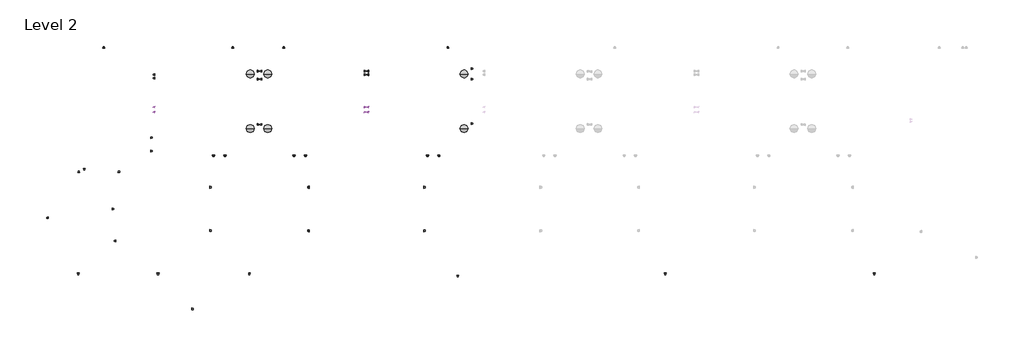
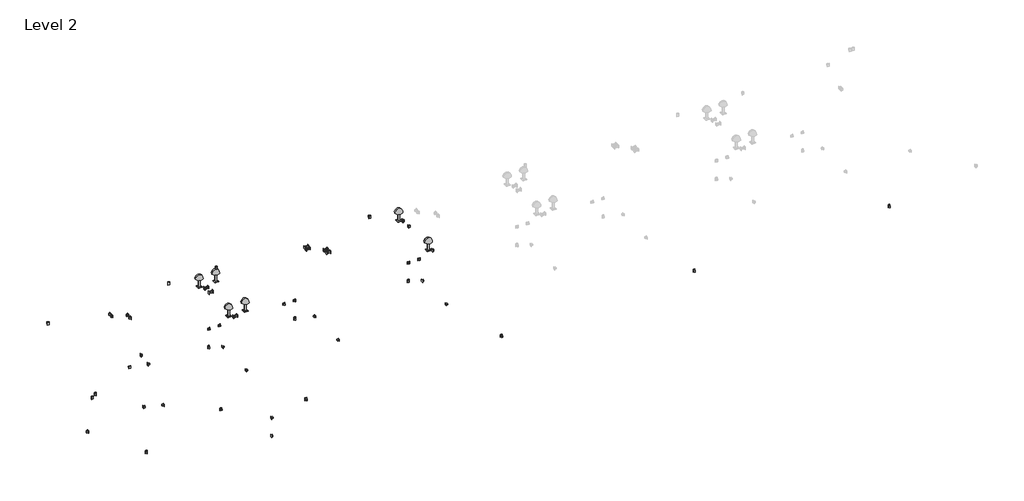
# One storey, part 1 of 2: 40 proxies, 16 switching devices, 6 light fixtures.
# Revit data of these elements (continued)
# Type "Table Lamp - Hemispheric : 60W - 230V" (continued)
#   built-in parameter 1150137 = 1
#   Color Filter = 16777215
#   Ballast Number of Poles = 1
#   T.L. Material = Wood - Birch
#   Mount Material = Metal - Chrome
#   Load Classification = Lighting - Dwelling Unit
#   Shade Material = Glass - Frosted
#   Base Material = Wood - Birch
#   Dimming Lamp Color Temperature Shift = (empty or 0)
#   Default Elevation = 0
#   Wattage Comments = ""
# Type "Lighting Switches One Way : One Way Switch"
#   Type Mark = "Lighting Switches One Way"
#   Classification.OmniClass.21.Number = "21-04 50 40 10"
#   Classification.OmniClass.21.Description = "Lighting Control"
#   Classification.UniFormat.II.Description = "Lighting Control"
#   Classification.OmniClass.23.Number = "23-35 37 00"
#   Classification.OmniClass.23.Description = "Electrical Switches"
#   Classification.UniFormat.II.Number = "D5040.10"
#   COBie.Type.CreatedBy = "info@mma.ie"
#   COBie.Type.CreatedOn = "2017-07-25T10:15:16"
#   COBie.Type.Name = "Lighting Switches One Way"
#   COBie.Type.Category = "23-35 37 00 : Electrical Switches"
#   COBie.Type.Description = "Lighting Switches One Way_One Way Switch"
#   COBie.Type.AssetType = "Fixed"
#   COBie.Type.Manufacturer = ""
#   COBie.Type.ModelNumber = ""
#   Label = ""
#   Keynote = "26 36 13.A"
#   COBie.Type.ReplacementCost = 0
#   Switch Voltage [instance default] = 230 V
#   Default Elevation = 1200 mm
#   Apparent Load = 0 VA
#   1.W.S. Width = 86 mm
#   1.W.S. Height = 86 mm
#   1.W.S. Depth = 59 mm
#   COBie.Type = yes
#   Visibility 7 = no
#   Visibility 6 = no
#   Visibility 5 = yes
#   Visibility 4 = no
#   Visibility 3 = no
#   Visibility 2 = no
#   Visibility 1 = no
#   Ballast Number of Poles = 1
#   Load Classification = Other
#   1.W.S. Material = Metal - Chrome
# Type "Lighting Switches Two Way : Two Way Switch"
#   Type Mark = "Lighting Switches Two Way"
#   Classification.OmniClass.23.Number = "23-35 37 00"
#   Classification.OmniClass.23.Description = "Electrical Switches"
#   COBie.Type.CreatedBy = "info@mma.ie"
#   COBie.Type.CreatedOn = "2017-07-25T10:15:16"
#   COBie.Type.Name = "Lighting Switches Two Way"
#   COBie.Type.Category = "23-35 37 00 : Electrical Switches"
#   COBie.Type.Description = "Lighting Switches Two Way_Two Way Switch"
#   COBie.Type.AssetType = "Fixed"
#   COBie.Type.Manufacturer = ""
#   COBie.Type.ModelNumber = ""
#   Label = ""
#   Keynote = "26 36 13.B"
#   COBie.Type.ReplacementCost = 0
#   Switch Voltage [instance default] = 230 V
#   Default Elevation = 1200 mm
#   Apparent Load = 0 VA
#   2.W.S. Width = 86 mm
#   2.W.S. Height = 86 mm
#   2.W.S. Depth = 59 mm
#   COBie.Type = yes
#   Visibility 7 = no
#   Visibility 6 = no
#   Visibility 5 = yes
#   Visibility 4 = no
#   Visibility 3 = no
#   Visibility 2 = no
#   Visibility 1 = no
#   Ballast Number of Poles = 1
#   Load Classification = Other
#   2.W.S. Material = Metal - Chrome
# Element 1 (IfcBuildingElementProxy, "M_Duplex Receptacle - Top Switched : Standard")
#   Mark = "7"
#   COBie.CreatedBy = "info@mma.ie"
#   COBie.CreatedOn = "2017-07-25T10:15:16"
#   COBie.Component.Name = "M_Duplex Receptacle - Top Switched_7"
#   COBie.Component.Space = "207"
#   COBie.Component.Description = "M_Duplex Receptacle - Top Switched: Standard"
#   Notes = "n/a"
#   COBie = yes
#   Phase Created = New Construction
# Element 2 (IfcBuildingElementProxy, "M_Duplex Receptacle - Top Switched : Standard")
#   Mark = "8"
#   COBie.CreatedBy = "info@mma.ie"
#   COBie.CreatedOn = "2017-07-25T10:15:16"
#   COBie.Component.Name = "M_Duplex Receptacle - Top Switched_8"
#   COBie.Component.Space = "207"
#   COBie.Component.Description = "M_Duplex Receptacle - Top Switched: Standard"
#   Notes = "n/a"
#   COBie = yes
#   Phase Created = New Construction
# Element 3 (IfcBuildingElementProxy, "M_Duplex Receptacle - Top Switched : Standard")
#   Mark = "9"
#   COBie.CreatedBy = "info@mma.ie"
#   COBie.CreatedOn = "2017-07-25T10:15:16"
#   COBie.Component.Name = "M_Duplex Receptacle - Top Switched_9"
#   COBie.Component.Space = "205"
#   COBie.Component.Description = "M_Duplex Receptacle - Top Switched: Standard"
#   Notes = "n/a"
#   COBie = yes
#   Phase Created = New Construction
# Element 4 (IfcBuildingElementProxy, "M_Duplex Receptacle - Top Switched : Standard")
#   Mark = "10"
#   COBie.CreatedBy = "info@mma.ie"
#   COBie.CreatedOn = "2017-07-25T10:15:16"
#   COBie.Component.Name = "M_Duplex Receptacle - Top Switched_10"
#   COBie.Component.Space = "205"
#   COBie.Component.Description = "M_Duplex Receptacle - Top Switched: Standard"
#   Notes = "n/a"
#   COBie = yes
#   Phase Created = New Construction
# Element 5 (IfcBuildingElementProxy, "M_Duplex Receptacle - Top Switched : Standard")
#   Mark = "15"
#   COBie.CreatedBy = "info@mma.ie"
#   COBie.CreatedOn = "2017-07-25T10:15:16"
#   COBie.Component.Name = "M_Duplex Receptacle - Top Switched_15"
#   COBie.Component.Space = "203"
#   COBie.Component.Description = "M_Duplex Receptacle - Top Switched: Standard"
#   Notes = "n/a"
#   COBie = yes
#   Phase Created = New Construction
# Element 6 (IfcBuildingElementProxy, "M_Duplex Receptacle - Top Switched : Standard")
#   Mark = "16"
#   COBie.CreatedBy = "info@mma.ie"
#   COBie.CreatedOn = "2017-07-25T10:15:16"
#   COBie.Component.Name = "M_Duplex Receptacle - Top Switched_16"
#   COBie.Component.Space = "203"
#   COBie.Component.Description = "M_Duplex Receptacle - Top Switched: Standard"
#   Notes = "n/a"
#   COBie = yes
#   Phase Created = New Construction
# Element 7 (IfcBuildingElementProxy, "M_Receptacle - 220V : Standard")
#   Mark = "15"
#   COBie.CreatedBy = "info@mma.ie"
#   COBie.CreatedOn = "2017-07-25T10:15:16"
#   COBie.Component.Name = "M_Receptacle - 220V_15"
#   COBie.Component.Space = "207"
#   COBie.Component.Description = "M_Receptacle - 220V: Standard"
#   Notes = "n/a"
#   COBie = yes
#   Phase Created = New Construction
# Element 8 (IfcBuildingElementProxy, "M_Receptacle - 220V : Standard")
#   Mark = "16"
#   COBie.CreatedBy = "info@mma.ie"
#   COBie.CreatedOn = "2017-07-25T10:15:16"
#   COBie.Component.Name = "M_Receptacle - 220V_16"
#   COBie.Component.Space = "207"
#   COBie.Component.Description = "M_Receptacle - 220V: Standard"
#   Notes = "n/a"
#   COBie = yes
#   Phase Created = New Construction
# Element 9 (IfcBuildingElementProxy, "M_Receptacle - 220V : Standard")
#   Mark = "17"
#   COBie.CreatedBy = "info@mma.ie"
#   COBie.CreatedOn = "2017-07-25T10:15:16"
#   COBie.Component.Name = "M_Receptacle - 220V_17"
#   COBie.Component.Space = "207"
#   COBie.Component.Description = "M_Receptacle - 220V: Standard"
#   Notes = "n/a"
#   COBie = yes
#   Phase Created = New Construction
# Element 10 (IfcBuildingElementProxy, "M_Receptacle - 220V : Standard")
#   Mark = "18"
#   COBie.CreatedBy = "info@mma.ie"
#   COBie.CreatedOn = "2017-07-25T10:15:16"
#   COBie.Component.Name = "M_Receptacle - 220V_18"
#   COBie.Component.Space = "207"
#   COBie.Component.Description = "M_Receptacle - 220V: Standard"
#   Notes = "n/a"
#   COBie = yes
#   Phase Created = New Construction
# Element 11 (IfcBuildingElementProxy, "M_Receptacle - 220V : Standard")
#   Mark = "19"
#   COBie.CreatedBy = "info@mma.ie"
#   COBie.CreatedOn = "2017-07-25T10:15:16"
#   COBie.Component.Name = "M_Receptacle - 220V_19"
#   COBie.Component.Space = "205"
#   COBie.Component.Description = "M_Receptacle - 220V: Standard"
#   Notes = "n/a"
#   COBie = yes
#   Phase Created = New Construction
# Element 12 (IfcBuildingElementProxy, "M_Receptacle - 220V : Standard")
#   Mark = "20"
#   COBie.CreatedBy = "info@mma.ie"
#   COBie.CreatedOn = "2017-07-25T10:15:16"
#   COBie.Component.Name = "M_Receptacle - 220V_20"
#   COBie.Component.Space = "203"
#   COBie.Component.Description = "M_Receptacle - 220V: Standard"
#   Notes = "n/a"
#   COBie = yes
#   Phase Created = New Construction
# Element 13 (IfcBuildingElementProxy, "M_Receptacle - 220V : Standard")
#   Mark = "21"
#   COBie.CreatedBy = "info@mma.ie"
#   COBie.CreatedOn = "2017-07-25T10:15:16"
#   COBie.Component.Name = "M_Receptacle - 220V_21"
#   COBie.Component.Space = "205"
#   COBie.Component.Description = "M_Receptacle - 220V: Standard"
#   Notes = "n/a"
#   COBie = yes
#   Phase Created = New Construction
# Element 14 (IfcBuildingElementProxy, "M_Receptacle - 220V : Standard")
#   Mark = "22"
#   COBie.CreatedBy = "info@mma.ie"
#   COBie.CreatedOn = "2017-07-25T10:15:16"
#   COBie.Component.Name = "M_Receptacle - 220V_22"
#   COBie.Component.Space = "203"
#   COBie.Component.Description = "M_Receptacle - 220V: Standard"
#   Notes = "n/a"
#   COBie = yes
#   Phase Created = New Construction
# Element 15 (IfcBuildingElementProxy, "M_Receptacle - 220V : Standard")
#   Comments = ""
#   Mark = "23"
#   COBie.CreatedBy = "info@mma.ie"
#   COBie.CreatedOn = "2017-07-25T10:15:16"
#   COBie.Component.Name = "M_Receptacle - 220V_23"
#   COBie.Component.Space = "202"
#   COBie.Component.Description = "M_Receptacle - 220V: Standard"
#   Notes = "n/a"
#   COBie = yes
#   Phase Created = New Construction
# Element 16 (IfcBuildingElementProxy, "M_Receptacle - 220V : Standard")
#   Mark = "24"
#   COBie.CreatedBy = "info@mma.ie"
#   COBie.CreatedOn = "2017-07-25T10:15:16"
#   COBie.Component.Name = "M_Receptacle - 220V_24"
#   COBie.Component.Space = "203"
#   COBie.Component.Description = "M_Receptacle - 220V: Standard"
#   Notes = "n/a"
#   COBie = yes
#   Phase Created = New Construction
# Element 17 (IfcBuildingElementProxy, "M_Receptacle - 220V : Standard")
#   Mark = "25"
#   COBie.CreatedBy = "info@mma.ie"
#   COBie.CreatedOn = "2017-07-25T10:15:16"
#   COBie.Component.Name = "M_Receptacle - 220V_25"
#   COBie.Component.Space = "203"
#   COBie.Component.Description = "M_Receptacle - 220V: Standard"
#   Notes = "n/a"
#   COBie = yes
#   Phase Created = New Construction
# Element 18 (IfcBuildingElementProxy, "M_Receptacle - 220V : Standard")
#   Comments = ""
#   Mark = "26"
#   COBie.CreatedBy = "info@mma.ie"
#   COBie.CreatedOn = "2017-07-25T10:15:16"
#   COBie.Component.Name = "M_Receptacle - 220V_26"
#   COBie.Component.Space = "202"
#   COBie.Component.Description = "M_Receptacle - 220V: Standard"
#   Notes = "n/a"
#   COBie = yes
#   Phase Created = New Construction
# Element 19 (IfcBuildingElementProxy, "M_Receptacle - 220V : Standard")
#   Comments = ""
#   Mark = "27"
#   COBie.CreatedBy = "info@mma.ie"
#   COBie.CreatedOn = "2017-07-25T10:15:16"
#   COBie.Component.Name = "M_Receptacle - 220V_27"
#   COBie.Component.Space = "202"
#   COBie.Component.Description = "M_Receptacle - 220V: Standard"
#   Notes = "n/a"
#   COBie = yes
#   Phase Created = New Construction
# Element 20 (IfcBuildingElementProxy, "M_Receptacle - 220V : Standard")
#   Mark = "28"
#   COBie.CreatedBy = "info@mma.ie"
#   COBie.CreatedOn = "2017-07-25T10:15:16"
#   COBie.Component.Name = "M_Receptacle - 220V_28"
#   COBie.Component.Space = "201"
#   COBie.Component.Description = "M_Receptacle - 220V: Standard"
#   Notes = "n/a"
#   COBie = yes
#   Phase Created = New Construction
# Element 21 (IfcBuildingElementProxy, "M_Receptacle - 220V : Standard")
#   Mark = "29"
#   COBie.CreatedBy = "info@mma.ie"
#   COBie.CreatedOn = "2017-07-25T10:15:16"
#   COBie.Component.Name = "M_Receptacle - 220V_29"
#   COBie.Component.Space = "201"
#   COBie.Component.Description = "M_Receptacle - 220V: Standard"
#   Notes = "n/a"
#   COBie = yes
#   Phase Created = New Construction
# Element 22 (IfcBuildingElementProxy, "M_Receptacle - 220V : Standard")
#   Mark = "30"
#   COBie.CreatedBy = "info@mma.ie"
#   COBie.CreatedOn = "2017-07-25T10:15:16"
#   COBie.Component.Name = "M_Receptacle - 220V_30"
#   COBie.Component.Space = "201"
#   COBie.Component.Description = "M_Receptacle - 220V: Standard"
#   Notes = "n/a"
#   COBie = yes
#   Phase Created = New Construction
# Element 23 (IfcBuildingElementProxy, "M_Receptacle - 220V : Standard")
#   Mark = "31"
#   COBie.CreatedBy = "info@mma.ie"
#   COBie.CreatedOn = "2017-07-25T10:15:16"
#   COBie.Component.Name = "M_Receptacle - 220V_31"
#   COBie.Component.Space = "201"
#   COBie.Component.Description = "M_Receptacle - 220V: Standard"
#   Notes = "n/a"
#   COBie = yes
#   Phase Created = New Construction
# Element 24 (IfcBuildingElementProxy, "M_Receptacle - 220V : Standard")
#   Mark = "32"
#   COBie.CreatedBy = "info@mma.ie"
#   COBie.CreatedOn = "2017-07-25T10:15:16"
#   COBie.Component.Name = "M_Receptacle - 220V_32"
#   COBie.Component.Space = "218"
#   COBie.Component.Description = "M_Receptacle - 220V: Standard"
#   Notes = "n/a"
#   COBie = yes
#   Phase Created = New Construction
# Element 25 (IfcBuildingElementProxy, "M_Receptacle - 220V : Standard")
#   Mark = "33"
#   COBie.CreatedBy = "info@mma.ie"
#   COBie.CreatedOn = "2017-07-25T10:15:16"
#   COBie.Component.Name = "M_Receptacle - 220V_33"
#   COBie.Component.Space = "217"
#   COBie.Component.Description = "M_Receptacle - 220V: Standard"
#   Notes = "n/a"
#   COBie = yes
#   Phase Created = New Construction
# Element 26 (IfcBuildingElementProxy, "M_Receptacle - 220V : Standard")
#   Mark = "34"
#   COBie.CreatedBy = "info@mma.ie"
#   COBie.CreatedOn = "2017-07-25T10:15:16"
#   COBie.Component.Name = "M_Receptacle - 220V_34"
#   COBie.Component.Space = "217"
#   COBie.Component.Description = "M_Receptacle - 220V: Standard"
#   Notes = "n/a"
#   COBie = yes
#   Phase Created = New Construction
# Element 27 (IfcBuildingElementProxy, "M_Receptacle - 220V : Standard")
#   Mark = "35"
#   COBie.CreatedBy = "info@mma.ie"
#   COBie.CreatedOn = "2017-07-25T10:15:16"
#   COBie.Component.Name = "M_Receptacle - 220V_35"
#   COBie.Component.Space = "217"
#   COBie.Component.Description = "M_Receptacle - 220V: Standard"
#   Notes = "n/a"
#   COBie = yes
#   Phase Created = New Construction
# Element 28 (IfcBuildingElementProxy, "M_Receptacle - 220V : Standard")
#   Mark = "36"
#   COBie.CreatedBy = "info@mma.ie"
#   COBie.CreatedOn = "2017-07-25T10:15:16"
#   COBie.Component.Name = "M_Receptacle - 220V_36"
#   COBie.Component.Space = "217"
#   COBie.Component.Description = "M_Receptacle - 220V: Standard"
#   Notes = "n/a"
#   COBie = yes
#   Phase Created = New Construction
# Element 29 (IfcBuildingElementProxy, "M_Receptacle - 220V : Standard")
#   Mark = "80"
#   COBie.CreatedBy = "info@mma.ie"
#   COBie.CreatedOn = "2017-07-25T10:15:16"
#   COBie.Component.Name = "M_Receptacle - 220V_80"
#   COBie.Component.Space = "205"
#   COBie.Component.Description = "M_Receptacle - 220V: Standard"
#   Notes = "n/a"
#   COBie = yes
#   Phase Created = New Construction
# Element 30 (IfcBuildingElementProxy, "M_Receptacle - 220V : Standard")
#   Mark = "81"
#   COBie.CreatedBy = "info@mma.ie"
#   COBie.CreatedOn = "2017-07-25T10:15:16"
#   COBie.Component.Name = "M_Receptacle - 220V_81"
#   COBie.Component.Space = "205"
#   COBie.Component.Description = "M_Receptacle - 220V: Standard"
#   Notes = "n/a"
#   COBie = yes
#   Phase Created = New Construction
# Element 31 (IfcBuildingElementProxy, "M_Receptacle - DATA socket : Standard")
#   Mark = "1"
#   COBie.CreatedBy = "info@mma.ie"
#   COBie.CreatedOn = "2017-07-25T10:15:16"
#   COBie.Component.Name = "M_Receptacle - DATA socket_1"
#   COBie.Component.Space = "203"
#   COBie.Component.Description = "M_Receptacle - DATA socket: Standard"
#   Notes = "n/a"
#   COBie = yes
#   Phase Created = New Construction
# Element 32 (IfcBuildingElementProxy, "M_Receptacle - DATA socket : Standard")
#   Comments = ""
#   Mark = "2"
#   COBie.CreatedBy = "info@mma.ie"
#   COBie.CreatedOn = "2017-07-25T10:15:16"
#   COBie.Component.Name = "M_Receptacle - DATA socket_2"
#   COBie.Component.Space = "202"
#   COBie.Component.Description = "M_Receptacle - DATA socket: Standard"
#   Notes = "n/a"
#   COBie = yes
#   Phase Created = New Construction
# Element 33 (IfcBuildingElementProxy, "M_Receptacle - DATA socket : Standard")
#   Mark = "3"
#   COBie.CreatedBy = "info@mma.ie"
#   COBie.CreatedOn = "2017-07-25T10:15:16"
#   COBie.Component.Name = "M_Receptacle - DATA socket_3"
#   COBie.Component.Space = "203"
#   COBie.Component.Description = "M_Receptacle - DATA socket: Standard"
#   Notes = "n/a"
#   COBie = yes
#   Phase Created = New Construction
# Element 34 (IfcBuildingElementProxy, "M_Receptacle - DATA socket : Standard")
#   Mark = "4"
#   COBie.CreatedBy = "info@mma.ie"
#   COBie.CreatedOn = "2017-07-25T10:15:16"
#   COBie.Component.Name = "M_Receptacle - DATA socket_4"
#   COBie.Component.Space = "205"
#   COBie.Component.Description = "M_Receptacle - DATA socket: Standard"
#   Notes = "n/a"
#   COBie = yes
#   Phase Created = New Construction
# Element 35 (IfcBuildingElementProxy, "M_Receptacle - DATA socket : Standard")
#   Mark = "5"
#   COBie.CreatedBy = "info@mma.ie"
#   COBie.CreatedOn = "2017-07-25T10:15:16"
#   COBie.Component.Name = "M_Receptacle - DATA socket_5"
#   COBie.Component.Space = "207"
#   COBie.Component.Description = "M_Receptacle - DATA socket: Standard"
#   Notes = "n/a"
#   COBie = yes
#   Phase Created = New Construction
# Element 36 (IfcBuildingElementProxy, "M_Receptacle - DATA socket : Standard")
#   Mark = "19"
#   COBie.CreatedBy = "info@mma.ie"
#   COBie.CreatedOn = "2017-07-25T10:15:16"
#   COBie.Component.Name = "M_Receptacle - DATA socket_19"
#   COBie.Component.Space = "205"
#   COBie.Component.Description = "M_Receptacle - DATA socket: Standard"
#   Notes = "n/a"
#   COBie = yes
#   Phase Created = New Construction
# Element 37 (IfcBuildingElementProxy, "M_Receptacle - DATA socket : Standard")
#   Mark = "20"
#   COBie.CreatedBy = "info@mma.ie"
#   COBie.CreatedOn = "2017-07-25T10:15:16"
#   COBie.Component.Name = "M_Receptacle - DATA socket_20"
#   COBie.Component.Space = "207"
#   COBie.Component.Description = "M_Receptacle - DATA socket: Standard"
#   Notes = "n/a"
#   COBie = yes
#   Phase Created = New Construction
# Element 38 (IfcBuildingElementProxy, "M_Receptacle -TV /Satellite Socket : Standard")
#   Mark = "1"
#   COBie.CreatedBy = "info@mma.ie"
#   COBie.CreatedOn = "2017-07-25T10:15:16"
#   COBie.Component.Name = "M_Receptacle -TV_1"
#   COBie.Component.Space = "207"
#   COBie.Component.Description = "M_Receptacle -TV: Standard"
#   Notes = "n/a"
#   COBie = yes
#   Phase Created = New Construction
# Element 39 (IfcBuildingElementProxy, "M_Receptacle -TV /Satellite Socket : Standard")
#   Mark = "2"
#   COBie.CreatedBy = "info@mma.ie"
#   COBie.CreatedOn = "2017-07-25T10:15:16"
#   COBie.Component.Name = "M_Receptacle -TV_2"
#   COBie.Component.Space = "203"
#   COBie.Component.Description = "M_Receptacle -TV: Standard"
#   Notes = "n/a"
#   COBie = yes
#   Phase Created = New Construction
# Element 40 (IfcBuildingElementProxy, "M_Receptacle -TV /Satellite Socket : Standard")
#   Mark = "7"
#   COBie.CreatedBy = "info@mma.ie"
#   COBie.CreatedOn = "2017-07-25T10:15:16"
#   COBie.Component.Name = "M_Receptacle -TV_7"
#   COBie.Component.Space = "205"
#   COBie.Component.Description = "M_Receptacle -TV: Standard"
#   Notes = "n/a"
#   COBie = yes
#   Phase Created = New Construction
# Element 41 (IfcLightFixture, "Table Lamp - Hemispheric : 60W - 230V")
#   Comments = "Lamps"
#   Mark = "5"
#   COBie.ExternalIdentifier = ""
#   COBie.CreatedBy = "info@mma.ie"
#   COBie.CreatedOn = "2017-07-25T10:15:16"
#   COBie.Component.Name = "Table Lamp - Hemispheric_5"
#   COBie.Component.Space = "207"
#   COBie.Component.Description = "Table Lamp - Hemispheric: 60W - 230V"
#   Notes = "n/a"
#   Floor Level = "Level 2"
#   COBie = yes
#   Phase Created = New Construction
#   Materials on its faces: "Metal - Chrome", "Glass - Frosted", "Wood - Birch"
# Element 42 (IfcLightFixture, "Table Lamp - Hemispheric : 60W - 230V")
#   Comments = "Lamps"
#   Mark = "6"
#   COBie.CreatedBy = "info@mma.ie"
#   COBie.CreatedOn = "2017-07-25T10:15:16"
#   COBie.Component.Name = "Table Lamp - Hemispheric_6"
#   COBie.Component.Space = "207"
#   COBie.Component.Description = "Table Lamp - Hemispheric: 60W - 230V"
#   Notes = "n/a"
#   Floor Level = "Level 2"
#   COBie = yes
#   Phase Created = New Construction
#   Materials on its faces: "Metal - Chrome", "Glass - Frosted", "Wood - Birch"
# Element 43 (IfcLightFixture, "Table Lamp - Hemispheric : 60W - 230V")
#   Comments = "Lamps"
#   Mark = "7"
#   COBie.CreatedBy = "info@mma.ie"
#   COBie.CreatedOn = "2017-07-25T10:15:16"
#   COBie.Component.Name = "Table Lamp - Hemispheric_7"
#   COBie.Component.Space = "205"
#   COBie.Component.Description = "Table Lamp - Hemispheric: 60W - 230V"
#   Notes = "n/a"
#   Floor Level = "Level 2"
#   COBie = yes
#   Phase Created = New Construction
#   Materials on its faces: "Metal - Chrome", "Glass - Frosted", "Wood - Birch"
# Element 44 (IfcLightFixture, "Table Lamp - Hemispheric : 60W - 230V")
#   Comments = "Lamps"
#   Mark = "8"
#   COBie.CreatedBy = "info@mma.ie"
#   COBie.CreatedOn = "2017-07-25T10:15:16"
#   COBie.Component.Name = "Table Lamp - Hemispheric_8"
#   COBie.Component.Space = "205"
#   COBie.Component.Description = "Table Lamp - Hemispheric: 60W - 230V"
#   Notes = "n/a"
#   Floor Level = "Level 2"
#   COBie = yes
#   Phase Created = New Construction
#   Materials on its faces: "Metal - Chrome", "Glass - Frosted", "Wood - Birch"
# Element 45 (IfcLightFixture, "Table Lamp - Hemispheric : 60W - 230V")
#   Comments = "Lamps"
#   Mark = "9"
#   COBie.CreatedBy = "info@mma.ie"
#   COBie.CreatedOn = "2017-07-25T10:15:16"
#   COBie.Component.Name = "Table Lamp - Hemispheric_9"
#   COBie.Component.Space = "203"
#   COBie.Component.Description = "Table Lamp - Hemispheric: 60W - 230V"
#   Notes = "n/a"
#   Floor Level = "Level 2"
#   COBie = yes
#   Phase Created = New Construction
#   Materials on its faces: "Metal - Chrome", "Glass - Frosted", "Wood - Birch"
# Element 46 (IfcLightFixture, "Table Lamp - Hemispheric : 60W - 230V")
#   Comments = "Lamps"
#   Mark = "10"
#   COBie.CreatedBy = "info@mma.ie"
#   COBie.CreatedOn = "2017-07-25T10:15:16"
#   COBie.Component.Name = "Table Lamp - Hemispheric_10"
#   COBie.Component.Space = "203"
#   COBie.Component.Description = "Table Lamp - Hemispheric: 60W - 230V"
#   Notes = "n/a"
#   Floor Level = "Level 2"
#   COBie = yes
#   Phase Created = New Construction
#   Materials on its faces: "Metal - Chrome", "Glass - Frosted", "Wood - Birch"
# Element 47 (IfcSwitchingDevice, "Lighting Switches One Way : One Way Switch")
#   Comments = "Switch"
#   Mark = "7"
#   COBie.CreatedBy = "info@mma.ie"
#   COBie.CreatedOn = "2017-07-25T10:15:16"
#   COBie.Component.Name = "Lighting Switches One Way_7"
#   COBie.Component.Space = "217"
#   COBie.Component.Description = "Lighting Switches One Way: One Way Switch"
#   Notes = "n/a"
#   Floor Level = "Level 2"
#   COBie = yes
#   Phase Created = New Construction
# Element 48 (IfcSwitchingDevice, "Lighting Switches One Way : One Way Switch")
#   Comments = "Switch"
#   Mark = "8"
#   COBie.CreatedBy = "info@mma.ie"
#   COBie.CreatedOn = "2017-07-25T10:15:16"
#   COBie.Component.Name = "Lighting Switches One Way_8"
#   COBie.Component.Space = "217"
#   COBie.Component.Description = "Lighting Switches One Way: One Way Switch"
#   Notes = "n/a"
#   Floor Level = "Level 2"
#   COBie = yes
#   Phase Created = New Construction
# Element 49 (IfcSwitchingDevice, "Lighting Switches One Way : One Way Switch")
#   Comments = "Switch"
#   Mark = "9"
#   COBie.CreatedBy = "info@mma.ie"
#   COBie.CreatedOn = "2017-07-25T10:15:16"
#   COBie.Component.Name = "Lighting Switches One Way_9"
#   COBie.Component.Space = "203"
#   COBie.Component.Description = "Lighting Switches One Way: One Way Switch"
#   Notes = "n/a"
#   Floor Level = "Level 2"
#   COBie = yes
#   Phase Created = New Construction
# Element 50 (IfcSwitchingDevice, "Lighting Switches One Way : One Way Switch")
#   Comments = "Switch"
#   Mark = "14"
#   COBie.CreatedBy = "info@mma.ie"
#   COBie.CreatedOn = "2017-07-25T10:15:16"
#   COBie.Component.Name = "Lighting Switches One Way_14"
#   COBie.Component.Space = "207"
#   COBie.Component.Description = "Lighting Switches One Way: One Way Switch"
#   Notes = "n/a"
#   Floor Level = "Level 2"
#   COBie = yes
#   Phase Created = New Construction
# Element 51 (IfcSwitchingDevice, "Lighting Switches One Way : One Way Switch")
#   Comments = "Switch"
#   Mark = "15"
#   COBie.CreatedBy = "info@mma.ie"
#   COBie.CreatedOn = "2017-07-25T10:15:16"
#   COBie.Component.Name = "Lighting Switches One Way_15"
#   COBie.Component.Space = "205"
#   COBie.Component.Description = "Lighting Switches One Way: One Way Switch"
#   Notes = "n/a"
#   Floor Level = "Level 2"
#   COBie = yes
#   Phase Created = New Construction
# Element 52 (IfcSwitchingDevice, "Lighting Switches One Way : One Way Switch")
#   Comments = "Switch"
#   Mark = "21"
#   COBie.CreatedBy = "info@mma.ie"
#   COBie.CreatedOn = "2017-07-25T10:15:16"
#   COBie.Component.Name = "Lighting Switches One Way_21"
#   COBie.Component.Space = "207"
#   COBie.Component.Description = "Lighting Switches One Way: One Way Switch"
#   Notes = "n/a"
#   Floor Level = "Level 2"
#   COBie = yes
#   Phase Created = New Construction
# Element 53 (IfcSwitchingDevice, "Lighting Switches One Way : One Way Switch")
#   Comments = "Switch"
#   Mark = "22"
#   COBie.CreatedBy = "info@mma.ie"
#   COBie.CreatedOn = "2017-07-25T10:15:16"
#   COBie.Component.Name = "Lighting Switches One Way_22"
#   COBie.Component.Space = "207"
#   COBie.Component.Description = "Lighting Switches One Way: One Way Switch"
#   Notes = "n/a"
#   Floor Level = "Level 2"
#   COBie = yes
#   Phase Created = New Construction
# Element 54 (IfcSwitchingDevice, "Lighting Switches One Way : One Way Switch")
#   Comments = "Switch"
#   Mark = "23"
#   COBie.CreatedBy = "info@mma.ie"
#   COBie.CreatedOn = "2017-07-25T10:15:16"
#   COBie.Component.Name = "Lighting Switches One Way_23"
#   COBie.Component.Space = "205"
#   COBie.Component.Description = "Lighting Switches One Way: One Way Switch"
#   Notes = "n/a"
#   Floor Level = "Level 2"
#   COBie = yes
#   Phase Created = New Construction
# Element 55 (IfcSwitchingDevice, "Lighting Switches One Way : One Way Switch")
#   Comments = "Switch"
#   Mark = "24"
#   COBie.CreatedBy = "info@mma.ie"
#   COBie.CreatedOn = "2017-07-25T10:15:16"
#   COBie.Component.Name = "Lighting Switches One Way_24"
#   COBie.Component.Space = "203"
#   COBie.Component.Description = "Lighting Switches One Way: One Way Switch"
#   Notes = "n/a"
#   Floor Level = "Level 2"
#   COBie = yes
#   Phase Created = New Construction
# Element 56 (IfcSwitchingDevice, "Lighting Switches One Way : One Way Switch")
#   Comments = "Switch"
#   Mark = "25"
#   COBie.CreatedBy = "info@mma.ie"
#   COBie.CreatedOn = "2017-07-25T10:15:16"
#   COBie.Component.Name = "Lighting Switches One Way_25"
#   COBie.Component.Space = "203"
#   COBie.Component.Description = "Lighting Switches One Way: One Way Switch"
#   Notes = "n/a"
#   Floor Level = "Level 2"
#   COBie = yes
#   Phase Created = New Construction
# Element 57 (IfcSwitchingDevice, "Lighting Switches One Way : One Way Switch")
#   Comments = "Switch"
#   Mark = "26"
#   COBie.CreatedBy = "info@mma.ie"
#   COBie.CreatedOn = "2017-07-25T10:15:16"
#   COBie.Component.Name = "Lighting Switches One Way_26"
#   COBie.Component.Space = "205"
#   COBie.Component.Description = "Lighting Switches One Way: One Way Switch"
#   Notes = "n/a"
#   Floor Level = "Level 2"
#   COBie = yes
#   Phase Created = New Construction
# Element 58 (IfcSwitchingDevice, "Lighting Switches One Way : One Way Switch")
#   Comments = "Switch"
#   Mark = "27"
#   COBie.CreatedBy = "info@mma.ie"
#   COBie.CreatedOn = "2017-07-25T10:15:16"
#   COBie.Component.Name = "Lighting Switches One Way_27"
#   COBie.Component.Space = "207"
#   COBie.Component.Description = "Lighting Switches One Way: One Way Switch"
#   Notes = "n/a"
#   Floor Level = "Level 2"
#   COBie = yes
#   Phase Created = New Construction
# Element 59 (IfcSwitchingDevice, "Lighting Switches One Way : One Way Switch")
#   Comments = "Switch"
#   Mark = "5"
#   COBie.CreatedBy = "info@mma.ie"
#   COBie.CreatedOn = "2017-07-25T10:15:16"
#   COBie.Component.Name = "Lighting Switches One Way_5"
#   COBie.Component.Space = "205"
#   COBie.Component.Description = "Lighting Switches One Way: One Way Switch"
#   Notes = "n/a"
#   Floor Level = "Level 2"
#   COBie = yes
#   Phase Created = New Construction
# Element 60 (IfcSwitchingDevice, "Lighting Switches One Way : One Way Switch")
#   Comments = "Switch"
#   Mark = "1"
#   COBie.CreatedBy = "info@mma.ie"
#   COBie.CreatedOn = "2017-07-25T10:15:16"
#   COBie.Component.Name = "Lighting Switches One Way_1"
#   COBie.Component.Space = "203"
#   COBie.Component.Description = "Lighting Switches One Way: One Way Switch"
#   Notes = "n/a"
#   Floor Level = "Level 2"
#   COBie = yes
#   Phase Created = New Construction
# Element 61 (IfcSwitchingDevice, "Lighting Switches Two Way : Two Way Switch")
#   Comments = "Switch"
#   Mark = "3"
#   COBie.CreatedBy = "info@mma.ie"
#   COBie.CreatedOn = "2017-07-25T10:15:16"
#   COBie.Component.Name = "Lighting Switches Two Way_3"
#   COBie.Component.Space = "217"
#   COBie.Component.Description = "Lighting Switches Two Way: Two Way Switch"
#   Notes = "n/a"
#   Floor Level = "Level 2"
#   COBie = yes
#   Phase Created = New Construction
# Element 62 (IfcSwitchingDevice, "Lighting Switches Two Way : Two Way Switch")
#   Mark = "6"
#   COBie.CreatedBy = "info@mma.ie"
#   COBie.CreatedOn = "2017-07-25T10:15:16"
#   COBie.Component.Name = "Lighting Switches Two Way_6"
#   COBie.Component.Space = "218"
#   COBie.Component.Description = "Lighting Switches Two Way: Two Way Switch"
#   Notes = "n/a"
#   Switch Voltage = 230 V
#   COBie = yes
#   Phase Created = New Construction
# Materials
#   "Stainless Steel": class "Metal", colour RGB 120 120 120, transparency 0, Description = "Stainless Steel 18/8", Cost = 0
#   "Wood - Birch": class "Wood", colour RGB 224 178 126, transparency 0
#   "Metal - Chrome": class "Metal", colour RGB 17 17 17, transparency 0, Comments = "Rendering appearance not upgraded "
#   "Glass - Frosted": class "Glass", colour RGB 250 244 225, transparency 0.55
# Space at (18637.696, 3108.313) mm, phase "New Construction", upper level "Level 3 Roof LP", upper offset 0 mm, lower offset 0 mm
#   Number = "220"
#   Name = "Roof Space Level 2"
#   Classification.Space.Number = "13-69 13"
#   Classification.Space.Description = "Roof Terrace"
#   COBie.CreatedBy = "info@mma.ie"
#   COBie.CreatedOn = "2017-07-25T10:15:16"
#   COBie.Space.Name = "220"
#   COBie.Space.Category = "13-69 13 : Roof Terraces"
#   COBie.Space.Description = "Roof Terrace"
#   Actual Lighting Load per area = 0
#   Actual Power Load per area = 0
#   Sensible Heat Gain per person = 0
#   Specified Lighting Load = 0
#   Specified Power Load = 0
#   Latent Heat Gain per person = 0
#   Total Heat Gain per person = 0
#   Area per Person = 0
#   Number of People = 4.57466 (stored number, unit not read)
#   COBie.Space.UsableHeight = 3500 mm
#   COBie.Space.GrossArea = 129.461 m²
#   COBie.Space.NetArea = 0 m²
#   Lighting Load Units = 0
#   Power Load Units = 0
#   Return Airflow = 0
#   Occupancy Unit = -1
#   Condition Type = 2
#   COBie = yes
#   Construction Type = none
# Space at (13915.849, 12217.839) mm, phase "New Construction", upper level "Level 3 Roof LP", upper offset 0 mm, lower offset 0 mm
#   Number = "207"
#   Name = "Bedroom"
#   Classification.Space.Number = "13-65 19"
#   Classification.Space.Description = "Bedroom"
#   COBie.CreatedBy = "info@mma.ie"
#   COBie.CreatedOn = "2017-07-25T10:15:16"
#   COBie.Space.Name = "207"
#   COBie.Space.Category = "13-65 19 : Bedroom"
#   COBie.Space.Description = "Bedroom"
#   Actual Lighting Load per area = 0
#   Actual Power Load per area = 0
#   Sensible Heat Gain per person = 0
#   Specified Lighting Load = 0
#   Specified Power Load = 0
#   Latent Heat Gain per person = 0
#   Total Heat Gain per person = 0
#   Area per Person = 0
#   Number of People = 0.749181 (stored number, unit not read)
#   COBie.Space.UsableHeight = 3500 mm
#   COBie.Space.GrossArea = 21.4052 m²
#   COBie.Space.NetArea = 0 m²
#   Lighting Load Units = 0
#   Power Load Units = 0
#   Return Airflow = 0
#   Occupancy Unit = -1
#   Condition Type = 2
#   COBie = yes
#   Construction Type = none
# Space at (18749.973, 12217.839) mm, phase "New Construction", upper level "Level 3 Roof LP", upper offset 0 mm, lower offset 0 mm
#   Number = "209"
#   Name = "Bedroom"
#   Classification.Space.Number = "13-65 19"
#   Classification.Space.Description = "Bedroom"
#   COBie.CreatedBy = "info@mma.ie"
#   COBie.CreatedOn = "2017-07-25T10:15:16"
#   COBie.Space.Name = "209"
#   COBie.Space.Category = "13-65 19 : Bedroom"
#   COBie.Space.Description = "Bedroom"
#   Actual Lighting Load per area = 0
#   Actual Power Load per area = 0
#   Sensible Heat Gain per person = 0
#   Specified Lighting Load = 0
#   Specified Power Load = 0
#   Latent Heat Gain per person = 0
#   Total Heat Gain per person = 0
#   Area per Person = 0
#   Number of People = 0.749459 (stored number, unit not read)
#   COBie.Space.UsableHeight = 3500 mm
#   COBie.Space.GrossArea = 21.4131 m²
#   COBie.Space.NetArea = 0 m²
#   Lighting Load Units = 0
#   Power Load Units = 0
#   Return Airflow = 0
#   Occupancy Unit = -1
#   Condition Type = 2
#   COBie = yes
#   Construction Type = none
# Space at (22421.249, 12383.96) mm, phase "New Construction", upper level "Level 3 Roof LP", upper offset 0 mm, lower offset 0 mm
#   Number = "211"
#   Name = "Bedroom"
#   Classification.Space.Number = "13-65 19"
#   Classification.Space.Description = "Bedroom"
#   COBie.CreatedBy = "info@mma.ie"
#   COBie.CreatedOn = "2017-07-25T10:15:16"
#   COBie.Space.Name = "211"
#   COBie.Space.Category = "13-65 19 : Bedroom"
#   COBie.Space.Description = "Bedroom"
#   Actual Lighting Load per area = 0
#   Actual Power Load per area = 0
#   Sensible Heat Gain per person = 0
#   Specified Lighting Load = 0
#   Specified Power Load = 0
#   Latent Heat Gain per person = 0
#   Total Heat Gain per person = 0
#   Area per Person = 0
#   Number of People = 0.749195 (stored number, unit not read)
#   COBie.Space.UsableHeight = 3510 mm
#   COBie.Space.GrossArea = 21.4056 m²
#   COBie.Space.NetArea = 0 m²
#   Lighting Load Units = 0
#   Power Load Units = 0
#   Return Airflow = 0
#   Occupancy Unit = -1
#   Condition Type = 2
#   COBie = yes
#   Construction Type = none
# Space at (2061.798, 12853.055) mm, phase "New Construction", upper level "Level 3 Roof LP", upper offset 0 mm, lower offset 0 mm
#   Number = "202"
#   Name = "Storage Room"
#   Classification.Space.Number = "13-63 13 11"
#   Classification.Space.Description = "Storage Room"
#   COBie.CreatedBy = "info@mma.ie"
#   COBie.CreatedOn = "2017-07-25T10:15:16"
#   COBie.Space.Name = "202"
#   COBie.Space.Category = "13-63 13 11 : Storage Room"
#   COBie.Space.Description = "Storage Room"
#   Actual Lighting Load per area = 0
#   Actual Power Load per area = 0
#   Sensible Heat Gain per person = 0
#   Specified Lighting Load = 0
#   Specified Power Load = 0
#   Latent Heat Gain per person = 0
#   Total Heat Gain per person = 0
#   Area per Person = 0
#   Number of People = 10.4646 (stored number, unit not read)
#   COBie.Space.UsableHeight = 3500 mm
#   COBie.Space.GrossArea = 17.1831 m²
#   COBie.Space.NetArea = 0 m²
#   Lighting Load Units = 0
#   Power Load Units = 0
#   Return Airflow = 0
#   Occupancy Unit = -1
#   Condition Type = 2
#   COBie = yes
#   Construction Type = none
# Space at (31042.934, 12915.548) mm, phase "New Construction", upper level "Level 3 Roof LP", upper offset 0 mm, lower offset 0 mm
#   Number = "215"
#   Name = "Bedroom"
#   Classification.Space.Number = "13-65 19"
#   Classification.Space.Description = "Bedroom"
#   COBie.CreatedBy = "info@mma.ie"
#   COBie.CreatedOn = "2017-07-25T10:15:16"
#   COBie.Space.Name = "215"
#   COBie.Space.Category = "13-65 19 : Bedroom"
#   COBie.Space.Description = "Bedroom"
#   Actual Lighting Load per area = 0
#   Actual Power Load per area = 0
#   Sensible Heat Gain per person = 0
#   Specified Lighting Load = 0
#   Specified Power Load = 0
#   Latent Heat Gain per person = 0
#   Total Heat Gain per person = 0
#   Area per Person = 0
#   Number of People = 0.951317 (stored number, unit not read)
#   COBie.Space.UsableHeight = 3500 mm
#   COBie.Space.GrossArea = 27.1805 m²
#   COBie.Space.NetArea = 0 m²
#   Lighting Load Units = 0
#   Power Load Units = 0
#   Return Airflow = 0
#   Occupancy Unit = -1
#   Condition Type = 2
#   COBie = yes
#   Construction Type = none
# Space at (26524.44, 12383.96) mm, phase "New Construction", upper level "Level 3 Roof LP", upper offset 0 mm, lower offset 0 mm
#   Number = "213"
#   Name = "Bedroom"
#   Classification.Space.Number = "13-65 19"
#   Classification.Space.Description = "Bedroom"
#   COBie.CreatedBy = "info@mma.ie"
#   COBie.CreatedOn = "2017-07-25T10:15:16"
#   COBie.Space.Name = "213"
#   COBie.Space.Category = "13-65 19 : Bedroom"
#   COBie.Space.Description = "Bedroom"
#   Actual Lighting Load per area = 0
#   Actual Power Load per area = 0
#   Sensible Heat Gain per person = 0
#   Specified Lighting Load = 0
#   Specified Power Load = 0
#   Latent Heat Gain per person = 0
#   Total Heat Gain per person = 0
#   Area per Person = 0
#   Number of People = 0.749192 (stored number, unit not read)
#   COBie.Space.UsableHeight = 3500 mm
#   COBie.Space.GrossArea = 21.4055 m²
#   COBie.Space.NetArea = 0 m²
#   Lighting Load Units = 0
#   Power Load Units = 0
#   Return Airflow = 0
#   Occupancy Unit = -1
#   Condition Type = 2
#   COBie = yes
#   Construction Type = none
# Space at (29215.602, 9759.247) mm, phase "New Construction", upper level "Level 3 Roof LP", upper offset 0 mm, lower offset 0 mm
#   Number = "216"
#   Name = "Bath"
#   Classification.Space.Number = "13-65 13"
#   Classification.Space.Description = "Bathroom"
#   COBie.CreatedBy = "info@mma.ie"
#   COBie.CreatedOn = "2017-07-25T10:15:16"
#   COBie.Space.Name = "216"
#   COBie.Space.Category = "13-65 13 : Bathroom"
#   COBie.Space.Description = "Bath"
#   Actual Lighting Load per area = 0
#   Actual Power Load per area = 0
#   Sensible Heat Gain per person = 0
#   Specified Lighting Load = 0
#   Specified Power Load = 0
#   Latent Heat Gain per person = 0
#   Total Heat Gain per person = 0
#   Area per Person = 0
#   Number of People = 0.150602 (stored number, unit not read)
#   COBie.Space.UsableHeight = 3500 mm
#   COBie.Space.GrossArea = 4.3029 m²
#   COBie.Space.NetArea = 0 m²
#   Lighting Load Units = 0
#   Power Load Units = 0
#   Return Airflow = 0
#   Occupancy Unit = -1
#   Condition Type = 2
#   COBie = yes
#   Construction Type = none
# Space at (27388.27, 9759.247) mm, phase "New Construction", upper level "Level 3 Roof LP", upper offset 0 mm, lower offset 0 mm
#   Number = "214"
#   Name = "Bath"
#   Classification.Space.Number = "13-65 13"
#   Classification.Space.Description = "Bathroom"
#   COBie.CreatedBy = "info@mma.ie"
#   COBie.CreatedOn = "2017-07-25T10:15:16"
#   COBie.Space.Name = "214"
#   COBie.Space.Category = "13-65 13 : Bathroom"
#   COBie.Space.Description = "Bath"
#   Actual Lighting Load per area = 0
#   Actual Power Load per area = 0
#   Sensible Heat Gain per person = 0
#   Specified Lighting Load = 0
#   Specified Power Load = 0
#   Latent Heat Gain per person = 0
#   Total Heat Gain per person = 0
#   Area per Person = 0
#   Number of People = 0.150111 (stored number, unit not read)
#   COBie.Space.UsableHeight = 3500 mm
#   COBie.Space.GrossArea = 4.28888 m²
#   COBie.Space.NetArea = 0 m²
#   Lighting Load Units = 0
#   Power Load Units = 0
#   Return Airflow = 0
#   Occupancy Unit = -1
#   Condition Type = 2
#   COBie = yes
#   Construction Type = none
# Space at (21251.303, 9875.532) mm, phase "New Construction", upper level "Level 3 Roof LP", upper offset 0 mm, lower offset 0 mm
#   Number = "212"
#   Name = "Bath"
#   Classification.Space.Number = "13-65 13"
#   Classification.Space.Description = "Bathroom"
#   COBie.CreatedBy = "info@mma.ie"
#   COBie.CreatedOn = "2017-07-25T10:15:16"
#   COBie.Space.Name = "212"
#   COBie.Space.Category = "13-65 13 : Bathroom"
#   COBie.Space.Description = "Bath"
#   Actual Lighting Load per area = 0
#   Actual Power Load per area = 0
#   Sensible Heat Gain per person = 0
#   Specified Lighting Load = 0
#   Specified Power Load = 0
#   Latent Heat Gain per person = 0
#   Total Heat Gain per person = 0
#   Area per Person = 0
#   Number of People = 0.150602 (stored number, unit not read)
#   COBie.Space.UsableHeight = 3500 mm
#   COBie.Space.GrossArea = 4.3029 m²
#   COBie.Space.NetArea = 0 m²
#   Lighting Load Units = 0
#   Power Load Units = 0
#   Return Airflow = 0
#   Occupancy Unit = -1
#   Condition Type = 2
#   COBie = yes
#   Construction Type = none
# Space at (19364.621, 9759.247) mm, phase "New Construction", upper level "Level 3 Roof LP", upper offset 0 mm, lower offset 0 mm
#   Number = "210"
#   Name = "Bath"
#   Classification.Space.Number = "13-65 13"
#   Classification.Space.Description = "Bathroom"
#   COBie.CreatedBy = "info@mma.ie"
#   COBie.CreatedOn = "2017-07-25T10:15:16"
#   COBie.Space.Name = "210"
#   COBie.Space.Category = "13-65 13 : Bathroom"
#   COBie.Space.Description = "Bath"
#   Actual Lighting Load per area = 0
#   Actual Power Load per area = 0
#   Sensible Heat Gain per person = 0
#   Specified Lighting Load = 0
#   Specified Power Load = 0
#   Latent Heat Gain per person = 0
#   Total Heat Gain per person = 0
#   Area per Person = 0
#   Number of People = 0.150111 (stored number, unit not read)
#   COBie.Space.UsableHeight = 3500 mm
#   COBie.Space.GrossArea = 4.28888 m²
#   COBie.Space.NetArea = 0 m²
#   Lighting Load Units = 0
#   Power Load Units = 0
#   Return Airflow = 0
#   Occupancy Unit = -1
#   Condition Type = 2
#   COBie = yes
#   Construction Type = none
# Space at (14995.637, 9875.532) mm, phase "New Construction", upper level "Level 3 Roof LP", upper offset 0 mm, lower offset 0 mm
#   Number = "208"
#   Name = "Bath"
#   Classification.Space.Number = "13-65 13"
#   Classification.Space.Description = "Bathroom"
#   COBie.CreatedBy = "info@mma.ie"
#   COBie.CreatedOn = "2017-07-25T10:15:16"
#   COBie.Space.Name = "208"
#   COBie.Space.Category = "13-65 13 : Bathroom"
#   COBie.Space.Description = "Bath"
#   Actual Lighting Load per area = 0
#   Actual Power Load per area = 0
#   Sensible Heat Gain per person = 0
#   Specified Lighting Load = 0
#   Specified Power Load = 0
#   Latent Heat Gain per person = 0
#   Total Heat Gain per person = 0
#   Area per Person = 0
#   Number of People = 0.150242 (stored number, unit not read)
#   COBie.Space.UsableHeight = 3500 mm
#   COBie.Space.GrossArea = 4.29263 m²
#   COBie.Space.NetArea = 0 m²
#   Lighting Load Units = 0
#   Power Load Units = 0
#   Return Airflow = 0
#   Occupancy Unit = -1
#   Condition Type = 2
#   COBie = yes
#   Construction Type = none
# Space at (8932.217, 9759.247) mm, phase "New Construction", upper level "Level 3 Roof LP", upper offset 0 mm, lower offset 0 mm
#   Number = "206"
#   Name = "Bath"
#   Classification.Space.Number = "13-65 13"
#   Classification.Space.Description = "Bathroom"
#   COBie.CreatedBy = "info@mma.ie"
#   COBie.CreatedOn = "2017-07-25T10:15:16"
#   COBie.Space.Name = "206"
#   COBie.Space.Category = "13-65 13 : Bathroom"
#   COBie.Space.Description = "Bath"
#   Actual Lighting Load per area = 0
#   Actual Power Load per area = 0
#   Sensible Heat Gain per person = 0
#   Specified Lighting Load = 0
#   Specified Power Load = 0
#   Latent Heat Gain per person = 0
#   Total Heat Gain per person = 0
#   Area per Person = 0
#   Number of People = 0.149872 (stored number, unit not read)
#   COBie.Space.UsableHeight = 3500 mm
#   COBie.Space.GrossArea = 4.28206 m²
#   COBie.Space.NetArea = 0 m²
#   Lighting Load Units = 0
#   Power Load Units = 0
#   Return Airflow = 0
#   Occupancy Unit = -1
#   Condition Type = 2
#   COBie = yes
#   Construction Type = none
# Space at (7237.782, 9875.532) mm, phase "New Construction", upper level "Level 3 Roof LP", upper offset 0 mm, lower offset 0 mm
#   Number = "204"
#   Name = "Bath"
#   Classification.Space.Number = "13-65 13"
#   Classification.Space.Description = "Bathroom"
#   COBie.CreatedBy = "info@mma.ie"
#   COBie.CreatedOn = "2017-07-25T10:15:16"
#   COBie.Space.Name = "204"
#   COBie.Space.Category = "13-65 13 : Bathroom"
#   COBie.Space.Description = "Bath"
#   Actual Lighting Load per area = 0
#   Actual Power Load per area = 0
#   Sensible Heat Gain per person = 0
#   Specified Lighting Load = 0
#   Specified Power Load = 0
#   Latent Heat Gain per person = 0
#   Total Heat Gain per person = 0
#   Area per Person = 0
#   Number of People = 0.15084 (stored number, unit not read)
#   COBie.Space.UsableHeight = 3500 mm
#   COBie.Space.GrossArea = 4.30971 m²
#   COBie.Space.NetArea = 0 m²
#   Lighting Load Units = 0
#   Power Load Units = 0
#   Return Airflow = 0
#   Occupancy Unit = -1
#   Condition Type = 2
#   COBie = yes
#   Construction Type = none
# Space at (1221.331, 8430.61) mm, phase "New Construction", upper level "Level 3 Roof LP", upper offset 0 mm, lower offset 0 mm
#   Number = "201"
#   Name = "Storage"
#   Classification.Space.Number = "13-63 13 11"
#   Classification.Space.Description = "Storage Room"
#   COBie.CreatedBy = "info@mma.ie"
#   COBie.CreatedOn = "2017-07-25T10:15:16"
#   COBie.Space.Name = "201"
#   COBie.Space.Category = "13-63 13 11 : Storage Room"
#   COBie.Space.Description = "Storage"
#   Actual Lighting Load per area = 0
#   Actual Power Load per area = 0
#   Sensible Heat Gain per person = 0
#   Specified Lighting Load = 0
#   Specified Power Load = 0
#   Latent Heat Gain per person = 0
#   Total Heat Gain per person = 0
#   Area per Person = 0
#   Number of People = 0.315247 (stored number, unit not read)
#   COBie.Space.UsableHeight = 3500 mm
#   COBie.Space.GrossArea = 9.00707 m²
#   COBie.Space.NetArea = 0 m²
#   Lighting Load Units = 0
#   Power Load Units = 0
#   Return Airflow = 0
#   Occupancy Unit = -1
#   Condition Type = 2
#   COBie = yes
#   Construction Type = none
# Space at (10016.539, 11622.722) mm, phase "New Construction", upper level "Level 3 Roof LP", upper offset 0 mm, lower offset 0 mm
#   Number = "205"
#   Name = "Bedroom"
#   Classification.Space.Number = "13-65 19"
#   Classification.Space.Description = "Bedroom"
#   COBie.CreatedBy = "info@mma.ie"
#   COBie.CreatedOn = "2017-07-25T10:15:16"
#   COBie.Space.Name = "205"
#   COBie.Space.Category = "13-65 19 : Bedroom"
#   COBie.Space.Description = "Bedroom"
#   Actual Lighting Load per area = 0
#   Actual Power Load per area = 0
#   Sensible Heat Gain per person = 0
#   Specified Lighting Load = 0
#   Specified Power Load = 0
#   Latent Heat Gain per person = 0
#   Total Heat Gain per person = 0
#   Area per Person = 0
#   Number of People = 0.749957 (stored number, unit not read)
#   COBie.Space.UsableHeight = 3500 mm
#   COBie.Space.GrossArea = 21.4273 m²
#   COBie.Space.NetArea = 0 m²
#   Lighting Load Units = 0
#   Power Load Units = 0
#   Return Airflow = 0
#   Occupancy Unit = -1
#   Condition Type = 2
#   COBie = yes
#   Construction Type = none
# Space at (11964.905, 7347.722) mm, phase "New Construction", upper level "Level 3 Roof LP", upper offset 0 mm, lower offset 0 mm
#   Number = "217"
#   Name = "Hall"
#   Classification.Space.Number = "13-25 11"
#   Classification.Space.Description = "Primary Circulation Spaces"
#   COBie.CreatedBy = "info@mma.ie"
#   COBie.CreatedOn = "2017-07-25T10:15:16"
#   COBie.Space.Name = "217"
#   COBie.Space.Category = "13-25 : Circulation Spaces"
#   COBie.Space.Description = "Hall"
#   Actual Lighting Load per area = 0
#   Actual Power Load per area = 0
#   Sensible Heat Gain per person = 0
#   Specified Lighting Load = 0
#   Specified Power Load = 0
#   Latent Heat Gain per person = 0
#   Total Heat Gain per person = 0
#   Area per Person = 0
#   Number of People = 1.45296 (stored number, unit not read)
#   COBie.Space.UsableHeight = 3500 mm
#   COBie.Space.GrossArea = 41.5133 m²
#   COBie.Space.NetArea = 0 m²
#   Lighting Load Units = 0
#   Power Load Units = 0
#   Return Airflow = 0
#   Occupancy Unit = -1
#   Condition Type = 2
#   COBie = yes
#   Construction Type = none
# Space at (6037.554, 11622.722) mm, phase "New Construction", upper level "Level 3 Roof LP", upper offset 0 mm, lower offset 0 mm
#   Number = "203"
#   Name = "Bedroom"
#   Classification.Space.Number = "13-65 19"
#   Classification.Space.Description = "Bedroom"
#   COBie.CreatedBy = "info@mma.ie"
#   COBie.CreatedOn = "2017-07-25T10:15:16"
#   COBie.Space.Name = "203"
#   COBie.Space.Category = "13-65 19 : Bedroom"
#   COBie.Space.Description = "Bedroom"
#   Actual Lighting Load per area = 0
#   Actual Power Load per area = 0
#   Sensible Heat Gain per person = 0
#   Specified Lighting Load = 0
#   Specified Power Load = 0
#   Latent Heat Gain per person = 0
#   Total Heat Gain per person = 0
#   Area per Person = 0
#   Number of People = 0.748431 (stored number, unit not read)
#   COBie.Space.UsableHeight = 3500 mm
#   COBie.Space.GrossArea = 21.3837 m²
#   COBie.Space.NetArea = 0 m²
#   Lighting Load Units = 0
#   Power Load Units = 0
#   Return Airflow = 0
#   Occupancy Unit = -1
#   Condition Type = 2
#   COBie = yes
#   Construction Type = none
# Space at (3775.005, 4237.539) mm, phase "New Construction", upper level "Level 3 Roof LP", upper offset 0 mm, lower offset 0 mm
#   Number = "218"
#   Name = "Stair 1"
#   Classification.Space.Number = "13-23 11 13"
#   Classification.Space.Description = "Stairway"
#   COBie.CreatedBy = "info@mma.ie"
#   COBie.CreatedOn = "2017-07-25T10:15:16"
#   COBie.Space.Name = "218"
#   COBie.Space.Category = "13-23 11 13 : Stairway"
#   COBie.Space.Description = "Stair 1"
#   Actual Lighting Load per area = 0
#   Actual Power Load per area = 0
#   Sensible Heat Gain per person = 0
#   Specified Lighting Load = 0
#   Specified Power Load = 0
#   Latent Heat Gain per person = 0
#   Total Heat Gain per person = 0
#   Area per Person = 0
#   Number of People = 0.447448 (stored number, unit not read)
#   COBie.Space.UsableHeight = 3500 mm
#   COBie.Space.GrossArea = 12.7842 m²
#   COBie.Space.NetArea = 0 m²
#   Lighting Load Units = 0
#   Power Load Units = 0
#   Return Airflow = 0
#   Occupancy Unit = -1
#   Condition Type = 2
#   COBie = yes
#   Construction Type = none
# Space at (33537.505, 9582.548) mm, phase "New Construction", upper level "Level 3 Roof LP", upper offset 0 mm, lower offset 0 mm
#   Number = "219"
#   Name = "Stair 2"
#   Classification.Space.Number = "13-23 11 13"
#   Classification.Space.Description = "Stairway"
#   COBie.CreatedBy = "info@mma.ie"
#   COBie.CreatedOn = "2017-07-25T10:15:16"
#   COBie.Space.Name = "219"
#   COBie.Space.Category = "13-23 11 13 : Stairway"
#   COBie.Space.Description = "Stair 2"
#   Actual Lighting Load per area = 0
#   Actual Power Load per area = 0
#   Sensible Heat Gain per person = 0
#   Specified Lighting Load = 0
#   Specified Power Load = 0
#   Latent Heat Gain per person = 0
#   Total Heat Gain per person = 0
#   Area per Person = 0
#   Number of People = 0.429399 (stored number, unit not read)
#   COBie.Space.UsableHeight = 3500 mm
#   COBie.Space.GrossArea = 12.2685 m²
#   COBie.Space.NetArea = 0 m²
#   Lighting Load Units = 0
#   Power Load Units = 0
#   Return Airflow = 0
#   Occupancy Unit = -1
#   Condition Type = 2
#   COBie = yes
#   Construction Type = none
